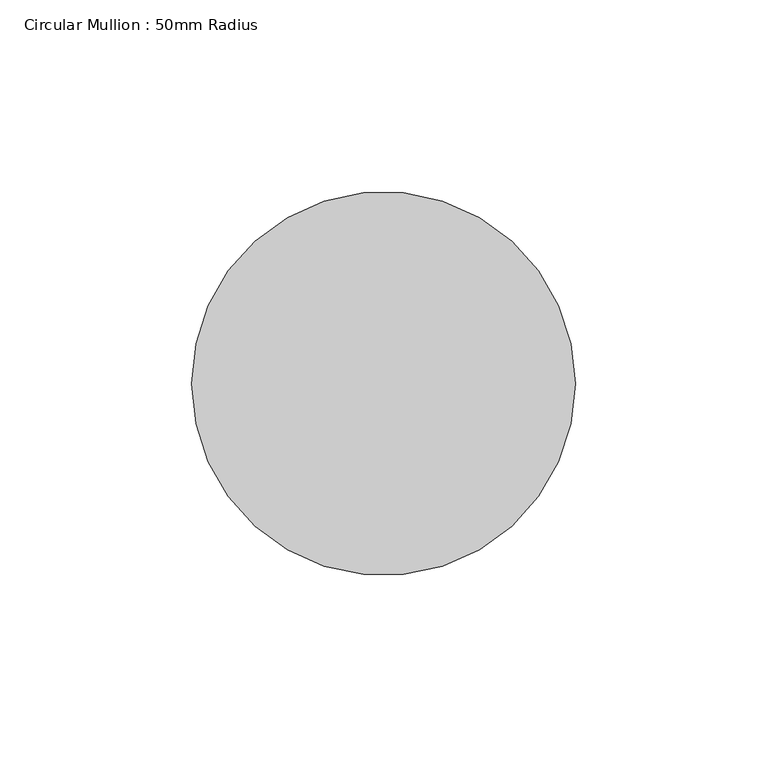
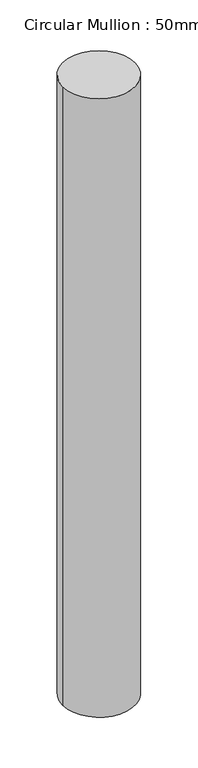
"""IFC4 building model written with IfcOpenShell, lengths in millimetres: member geometry, Circular Mullion : 50mm Radius."""

from ifc_helpers import new_model, si_unit, point, frame, origin, origin_2d, place, context, project, spatial, circle_curve, trimmed, segment, composite_curve, outline, extrude, source, transform, mapped, element, save


def circular_mullion_50mm_radius_7d8880af(model_context):
    return source(origin(), model_context, "Body", "SweptSolid", [
        extrude(outline(composite_curve([segment(trimmed(circle_curve(origin_2d(), 50.0), [point((50.0, 0.0))], [point((-50.0, 0.0))], False, "CARTESIAN"), True, "CONTINUOUS"), segment(trimmed(circle_curve(origin_2d(), 50.0), [point((-50.0, 0.0))], [point((50.0, 0.0))], False, "CARTESIAN"), True, "CONTINUOUS")], self_intersect=False)), frame((0.0, 0.0, -901.1325542), z_axis=(0.0, 0.0, 1.0), x_axis=(1.0, 0.0, 0.0)), (0.0, 0.0, 1.0), 901.1325542),
    ])


if __name__ == "__main__":
    model = new_model("IFC4")
    model_context = context("Model", 3, world=origin())
    ifc_project = project(units=[si_unit("LENGTHUNIT", "METRE", prefix="MILLI")], contexts=[model_context])
    site = spatial("IfcSite", under=ifc_project)
    building = spatial("IfcBuilding", under=site)
    placement = place(None, origin())
    circular_mullion_50mm_radius_shape = circular_mullion_50mm_radius_7d8880af(model_context)
    element("IfcMember", 1, ObjectType="Circular Mullion : 50mm Radius", at=placement, inside=building, context=model_context, shape_type="MappedRepresentation", body=[
        mapped(circular_mullion_50mm_radius_shape, transform((0.0, 0.0, 0.0), x_axis=(1.0, 0.0, 0.0), y_axis=(0.0, 1.0, 0.0), z_axis=(0.0, 0.0, 1.0))),
    ])
    save(model, "model.ifc")

# Revit data of these elements
# Type "Circular Mullion : 50mm Radius"
#   built-in parameter 1007350 = 0.164042 (stored number, unit not read)
# Element 1 (IfcMember, "Circular Mullion : 50mm Radius")
#   Materials on its faces: "Aluminium"
# Materials
#   "Aluminium": class "Metal", colour RGB 247 247 247, transparency 0, Description = "Aluminium 6061", Cost = 0
